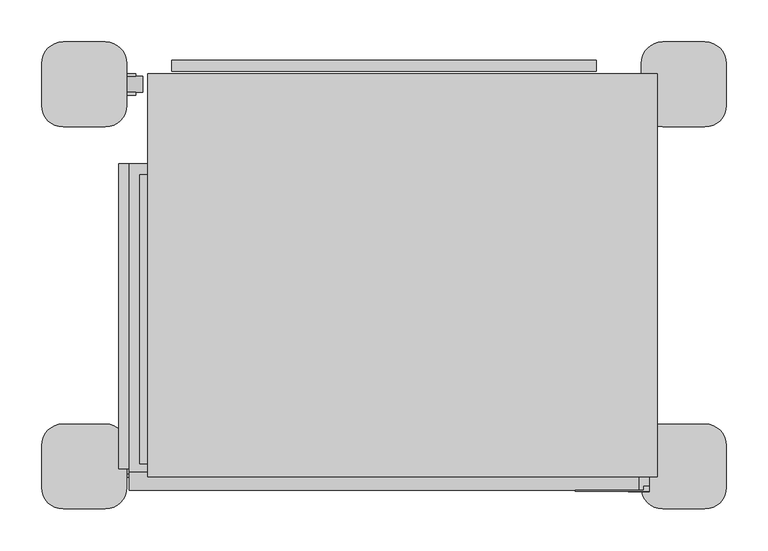
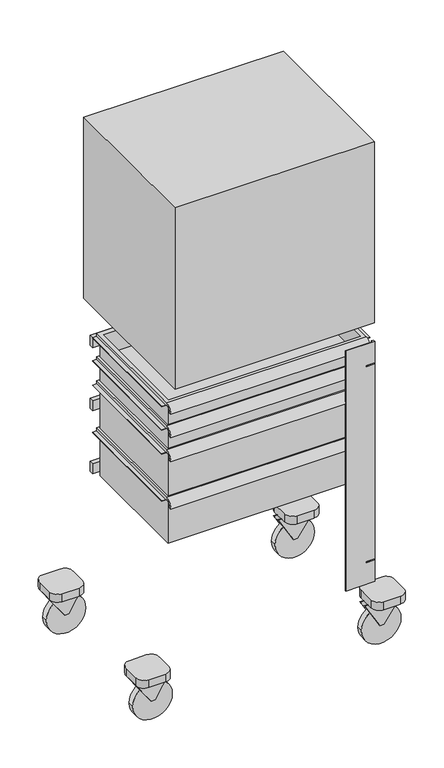
# IFC4 building model written with IfcOpenShell, lengths in millimetres: proxy geometry, M8185 - System, Stress Exercise, w-Treadmill : M8185 - System, Stress Exercise, w-Treadmill.
# Revit data of these elements (continued)
# Type "M8185 - System, Stress Exercise, w-Treadmill : M8185 - System, Stress Exercise, w-Treadmill" (continued)
#   ELEC_Phase1 = "1"
#   ELEC_HertzSwitch = "0"
#   ELEC_HertzDependent = "-1"
#   ELEC_Hertz = "60"
#   ELEC_Amps2 = "20"
#   ELEC_Amps1 = "20"
#   DetailDescription = "Stress exercise system with treadmill and respiratory/metabolic assessment. The system includes an ECG amplifier, chart recorder, display, console, treadmill and modules for respiratory/metabolic assessment. Used to determine patient's functional capacity, predict and diagnose cardiopulmonary and vascular diseases and for rehabilitation of patients b covering from leg injuries or other type of illness. Some vendors require a NEMA 5-20R non-locking receptacle for their treadmills."
#   CAT_VA = "C"
#   CAT_Navy = "C"
#   CAT_IHS = "-"
#   CAT_Army = "C"
#   CAT_AF = "C"
#   BTUperhour = "0"
#   Weight_IP = 520
#   DIM_Width_IP = 5' - 6"
#   DIM_Height_IP = 4' - 2"
#   DIM_Depth_IP = 7' - 6"
#   Assembly Code = ""
# Element 1 (IfcBuildingElementProxy, "M8185 - System, Stress Exercise, w-Treadmill : M8185 - System, Stress Exercise, w-Treadmill")
#   Location = "OPTM1"
#   Materials on its faces: "Finish LU Soft White", "EquipSpace", "Finish", "Wheel Material"
# Materials
#   "Finish LU Soft White": class "Plastic", colour RGB 245 239 218, transparency 0
#   "EquipSpace": class "Unassigned", colour RGB 221 217 195, transparency 0.5
#   "Finish": class "Plastic", colour RGB 245 239 218, transparency 0
#   "Wheel Material": class "Plastic", colour RGB 5 5 5, transparency 0
